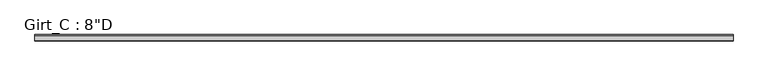
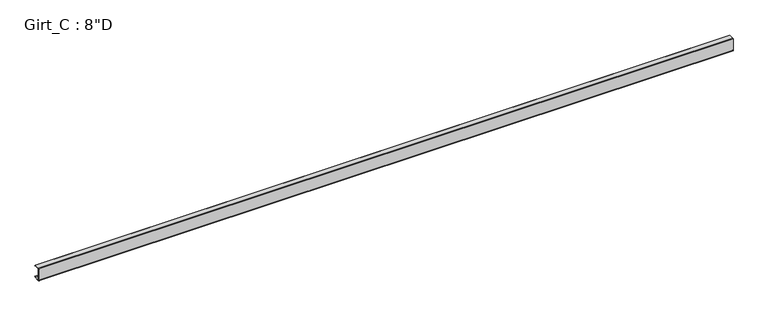
"""IFC4 building model written with IfcOpenShell, lengths in millimetres: beam geometry."""

from ifc_helpers import new_model, si_unit, point, frame, frame_2d, origin, place, context, project, spatial, polyline, circle_curve, trimmed, segment, composite_curve, outline, extrude, source, transform, mapped, element, save


def beam_b0195909(model_context):
    return source(origin(), model_context, "Body", "SweptSolid", [
        extrude(outline(composite_curve([segment(polyline([(87.5109375, 101.6), (99.7560415, 87.0068534), (97.6278742, 85.221109), (86.2154765, 98.821875), (3.3005807, 98.821875)]), True, "CONTINUOUS"), segment(trimmed(circle_curve(frame_2d((3.3741066, 96.8381931)), 1.9850441), [point((3.3005807, 98.821875))], [point((1.3890625, 96.8381931))], True, "CARTESIAN"), True, "CONTINUOUS"), segment(polyline([(1.3890625, 96.8381931), (1.3890625, -96.8389339)]), True, "CONTINUOUS"), segment(trimmed(circle_curve(frame_2d((3.3748024, -96.8389339)), 1.9857399), [point((1.3890625, -96.8389339))], [point((3.2694106, -98.821875))], True, "CARTESIAN"), True, "CONTINUOUS"), segment(polyline([(3.2694106, -98.821875), (86.2154765, -98.821875), (97.6510975, -85.1934327), (99.7792647, -86.979177), (87.5109375, -101.6), (3.3734375, -101.6)]), True, "CONTINUOUS"), segment(trimmed(circle_curve(frame_2d((3.3734375, -96.8375)), 4.7625), [point((3.3734375, -101.6))], [point((-1.3890625, -96.8375))], False, "CARTESIAN"), True, "CONTINUOUS"), segment(polyline([(-1.3890625, -96.8375), (-1.3890625, 96.8375)]), True, "CONTINUOUS"), segment(trimmed(circle_curve(frame_2d((3.3734375, 96.8375)), 4.7625), [point((-1.3890625, 96.8375))], [point((3.3734375, 101.6))], False, "CARTESIAN"), True, "CONTINUOUS"), segment(polyline([(3.3734375, 101.6), (87.5109375, 101.6)]), True, "CONTINUOUS")], self_intersect=False)), frame((-5554.9121796, 0.0, 0.0), z_axis=(1.0, 0.0, 0.0), x_axis=(0.0, 1.0, 0.0)), (0.0, 0.0, 1.0), 11010.9),
    ])


if __name__ == "__main__":
    model = new_model("IFC4")
    model_context = context("Model", 3, world=origin())
    ifc_project = project(units=[si_unit("LENGTHUNIT", "METRE", prefix="MILLI")], contexts=[model_context])
    site = spatial("IfcSite", under=ifc_project)
    building = spatial("IfcBuilding", under=site)
    placement = place(None, origin())
    beam_shape = beam_b0195909(model_context)
    element("IfcBeam", 1, ObjectType="Girt_C : 8\"D", at=placement, inside=building, context=model_context, shape_type="MappedRepresentation", body=[
        mapped(beam_shape, transform((0.0, 0.0, 0.0), x_axis=(1.0, 0.0, 0.0), y_axis=(0.0, 1.0, 0.0), z_axis=(0.0, 0.0, 1.0))),
    ])
    save(model, "model.ifc")

# Revit data of these elements
# Type "Girt_C : 8\"D"
#   half leg = 0' - 1 3/4"
#   Web_Thickness = 0' - 0 7/64"
#   Length [instance default] = 10' - 0"
#   Leg_1 = 0' - 3 1/2"
#   Height = 0' - 8"
#   Structural Material [instance default] = none
# Element 1 (IfcBeam, "Girt_C : 8\"D")
#   Structural Material = CEE' SECTION (8.0x3.5C - SEE STRUCT. DWGS)
#   Materials on its faces: "CEE' SECTION (8.0x3.5C - SEE STRUCT. DWGS)"
# Materials
#   "CEE' SECTION (8.0x3.5C - SEE STRUCT. DWGS)": class "Metal", colour RGB 137 146 153, transparency 0, Description = "Steel, mill finish", Cost = 0
